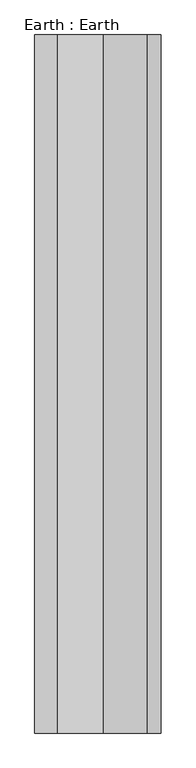
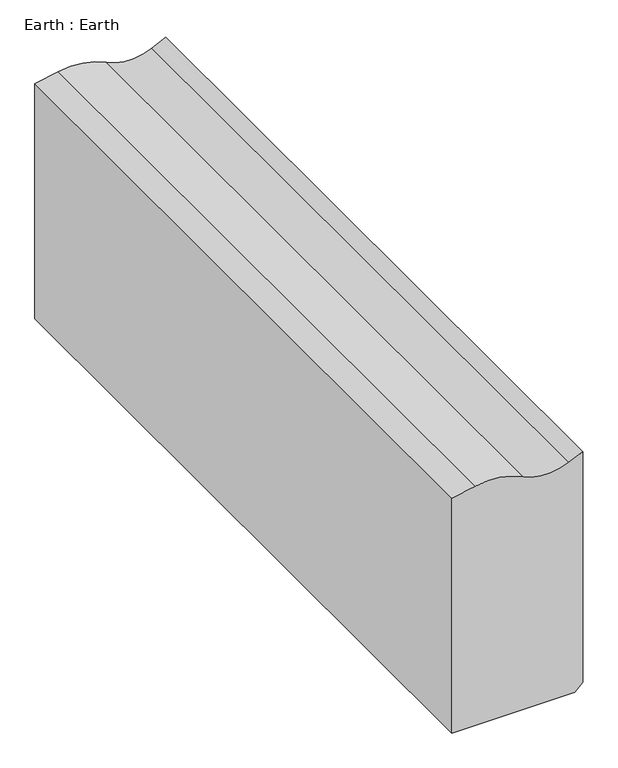
"""IFC4 building model written with IfcOpenShell, lengths in millimetres: proxy geometry, Earth : Earth."""

from ifc_helpers import new_model, si_unit, point, frame, frame_2d, origin, place, context, project, spatial, polyline, circle_curve, trimmed, segment, composite_curve, outline, extrude, source, transform, mapped, element, save


def earth_earth_1ffde3c4(model_context):
    return source(origin(), model_context, "Body", "SweptSolid", [
        extrude(outline(composite_curve([segment(polyline([(32620.9902343, -10057.5706312), (32620.9902343, -9717.2148439), (32643.1028304, -9695.1022478), (33318.0501956, -9695.1022478), (33300.0908366, -9733.8927957)]), True, "CONTINUOUS"), segment(trimmed(circle_curve(frame_2d((33431.3167137, -9794.6481283)), 144.607888), [point((33300.0908366, -9733.8927957))], [point((33302.6181918, -9860.5884932))], True, "CARTESIAN"), True, "CONTINUOUS"), segment(trimmed(circle_curve(frame_2d((33120.1913863, -9954.0572443)), 204.9779178), [point((33302.6181918, -9860.5884932))], [point((33321.4784396, -9992.7802216))], False, "CARTESIAN"), True, "CONTINUOUS"), segment(polyline([(33321.4784396, -9992.7802216), (33309.014262, -10057.5706312), (32620.9902343, -10057.5706312)]), True, "CONTINUOUS")], self_intersect=False)), frame((0.0, 7982.1531721, 0.0), z_axis=(0.0, 1.0, 0.0), x_axis=(0.0, 0.0, 1.0)), (0.0, 0.0, 1.0), 2000.0),
    ])


if __name__ == "__main__":
    model = new_model("IFC4")
    model_context = context("Model", 3, world=origin())
    ifc_project = project(units=[si_unit("LENGTHUNIT", "METRE", prefix="MILLI")], contexts=[model_context])
    site = spatial("IfcSite", under=ifc_project)
    building = spatial("IfcBuilding", under=site)
    placement = place(None, origin())
    earth_earth_shape = earth_earth_1ffde3c4(model_context)
    element("IfcBuildingElementProxy", 1, Name="Earth : Earth", ObjectType="Earth : Earth", at=placement, inside=building, context=model_context, shape_type="MappedRepresentation", body=[
        mapped(earth_earth_shape, transform((0.0, 0.0, 0.0), x_axis=(1.0, 0.0, 0.0), y_axis=(0.0, 1.0, 0.0), z_axis=(0.0, 0.0, 1.0))),
    ])
    save(model, "model.ifc")

# Revit data of these elements
# Type "Earth : Earth"
#   NameOverride = "Earth"
# Element 1 (IfcBuildingElementProxy, "Earth : Earth")
#   Materials on its faces: "GROUND SOIL"
# Materials
#   "GROUND SOIL": class "Unassigned", colour RGB 170 124 75, transparency 0, Cost = 0
